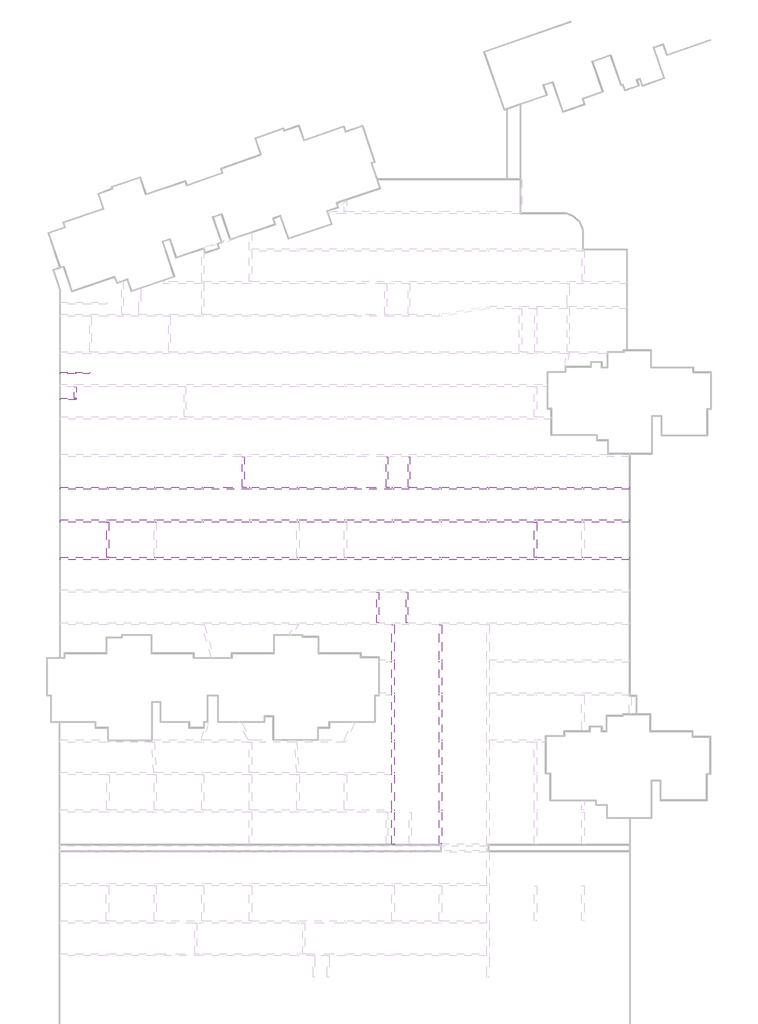
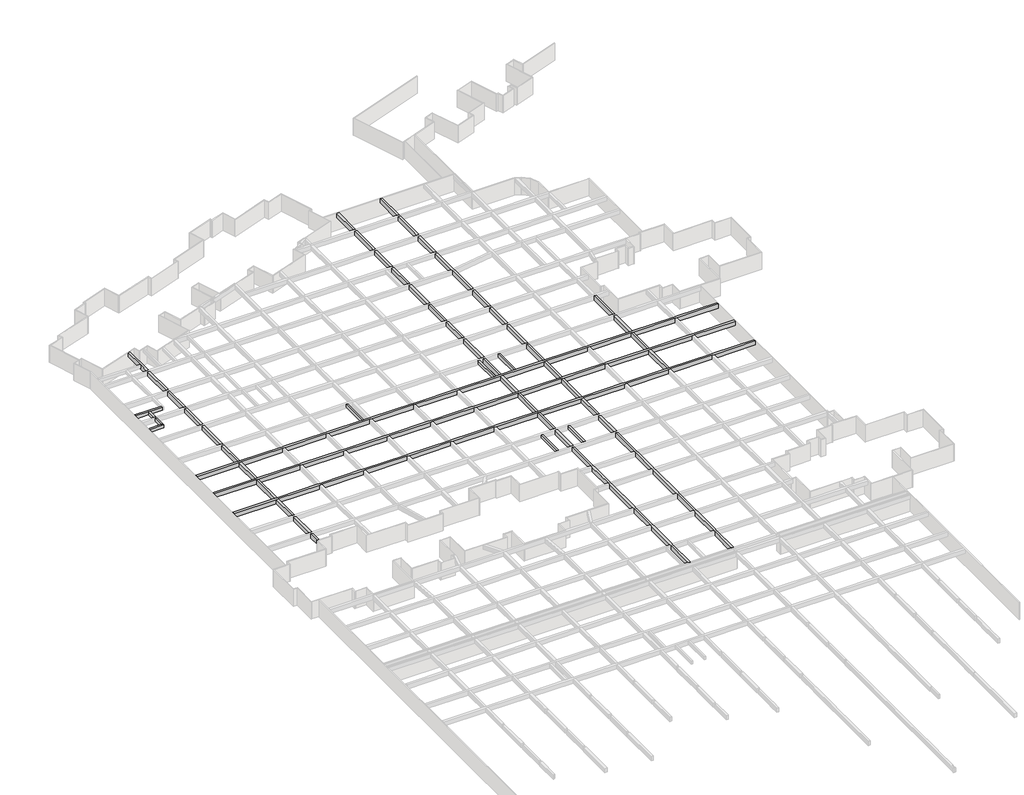
# One storey, part 12 of 14: 15 beams.
"""IFC4 building model written with IfcOpenShell, lengths in millimetres."""

from ifc_helpers import new_model, si_unit, frame, origin, place, context, project, spatial, polyline, outline, extrude, faceted_brep, element, save

model = new_model("IFC4")

# Units and contexts
model_context = context("Model", 3, world=origin())
ifc_project = project(units=[si_unit("LENGTHUNIT", "METRE", prefix="MILLI")], contexts=[model_context])

# Site, building, storey
site = spatial("IfcSite", under=ifc_project)
building = spatial("IfcBuilding", under=site)
storey = spatial("IfcBuildingStorey", under=building, Name="户型图", Elevation=0.0)

# Beams
placement = place(None, origin())
element("IfcBeam", 1, ObjectType="混凝土 - 矩形梁 : KL_beam", at=placement, inside=storey, context=model_context, shape_type="Brep", body=[
    faceted_brep([(-594019.2557706, -67959.4327531, 3300.0), (-594019.2557706, -68359.4327531, 3300.0), (-586267.6529954, -68359.4327531, 3300.0), (-585867.6529954, -68359.4327531, 3300.0), (-578267.6529954, -68359.4327531, 3300.0), (-577867.6529954, -68359.4327531, 3300.0), (-570267.6529954, -68359.4327531, 3300.0), (-569867.6529954, -68359.4327531, 3300.0), (-562267.6529954, -68359.4327531, 3300.0), (-561867.6529954, -68359.4327531, 3300.0), (-554267.6529954, -68359.4327531, 3300.0), (-553867.6529954, -68359.4327531, 3300.0), (-546267.6529954, -68359.4327531, 3300.0), (-545867.6529954, -68359.4327531, 3300.0), (-538267.6529954, -68359.4327531, 3300.0), (-537867.6529954, -68359.4327531, 3300.0), (-530267.6529954, -68359.4327531, 3300.0), (-529867.6529954, -68359.4327531, 3300.0), (-522267.6529954, -68359.4327531, 3300.0), (-521867.6529954, -68359.4327531, 3300.0), (-514267.6529954, -68359.4327531, 3300.0), (-513867.6529954, -68359.4327531, 3300.0), (-506267.6529954, -68359.4327531, 3300.0), (-505867.6529954, -68359.4327531, 3300.0), (-498277.6529954, -68359.4327531, 3300.0), (-498277.6529954, -67959.4327531, 3300.0), (-505867.6529954, -67959.4327531, 3300.0), (-506267.6529954, -67959.4327531, 3300.0), (-513867.6529954, -67959.4327531, 3300.0), (-514267.6529954, -67959.4327531, 3300.0), (-521867.6529954, -67959.4327531, 3300.0), (-522267.6529954, -67959.4327531, 3300.0), (-529867.6529954, -67959.4327531, 3300.0), (-530267.6529954, -67959.4327531, 3300.0), (-535217.6529954, -67959.4327531, 3300.0), (-535517.6529954, -67959.4327531, 3300.0), (-537867.6529954, -67959.4327531, 3300.0), (-538267.6529954, -67959.4327531, 3300.0), (-538917.6529954, -67959.4327531, 3300.0), (-539217.6529954, -67959.4327531, 3300.0), (-545867.6529954, -67959.4327531, 3300.0), (-546267.6529954, -67959.4327531, 3300.0), (-553867.6529954, -67959.4327531, 3300.0), (-554267.6529954, -67959.4327531, 3300.0), (-561867.6529954, -67959.4327531, 3300.0), (-562267.6529954, -67959.4327531, 3300.0), (-563117.6529954, -67959.4327531, 3300.0), (-563417.6529954, -67959.4327531, 3300.0), (-569867.6529954, -67959.4327531, 3300.0), (-570267.6529954, -67959.4327531, 3300.0), (-577867.6529954, -67959.4327531, 3300.0), (-578267.6529954, -67959.4327531, 3300.0), (-585867.6529954, -67959.4327531, 3300.0), (-586267.6529954, -67959.4327531, 3300.0), (-594019.2557706, -67959.4327531, 2500.0), (-498277.6529954, -67959.4327531, 2500.0), (-505867.6529954, -67959.4327531, 2500.0), (-506267.6529954, -67959.4327531, 2500.0), (-513867.6529954, -67959.4327531, 2500.0), (-514267.6529954, -67959.4327531, 2500.0), (-521867.6529954, -67959.4327531, 2500.0), (-522267.6529954, -67959.4327531, 2500.0), (-529867.6529954, -67959.4327531, 2500.0), (-530267.6529954, -67959.4327531, 2500.0), (-537867.6529954, -67959.4327531, 2500.0), (-538267.6529954, -67959.4327531, 2500.0), (-545867.6529954, -67959.4327531, 2500.0), (-546267.6529954, -67959.4327531, 2500.0), (-553867.6529954, -67959.4327531, 2500.0), (-554267.6529954, -67959.4327531, 2500.0), (-561867.6529954, -67959.4327531, 2500.0), (-562267.6529954, -67959.4327531, 2500.0), (-569867.6529954, -67959.4327531, 2500.0), (-570267.6529954, -67959.4327531, 2500.0), (-577867.6529954, -67959.4327531, 2500.0), (-578267.6529954, -67959.4327531, 2500.0), (-585867.6529954, -67959.4327531, 2500.0), (-586267.6529954, -67959.4327531, 2500.0), (-594019.2557706, -68359.4327531, 2500.0), (-498277.6529954, -68359.4327531, 2500.0), (-505867.6529954, -68359.4327531, 2500.0), (-506267.6529954, -68359.4327531, 2500.0), (-513867.6529954, -68359.4327531, 2500.0), (-514267.6529954, -68359.4327531, 2500.0), (-521867.6529954, -68359.4327531, 2500.0), (-522267.6529954, -68359.4327531, 2500.0), (-529867.6529954, -68359.4327531, 2500.0), (-530267.6529954, -68359.4327531, 2500.0), (-537867.6529954, -68359.4327531, 2500.0), (-538267.6529954, -68359.4327531, 2500.0), (-545867.6529954, -68359.4327531, 2500.0), (-546267.6529954, -68359.4327531, 2500.0), (-553867.6529954, -68359.4327531, 2500.0), (-554267.6529954, -68359.4327531, 2500.0), (-561867.6529954, -68359.4327531, 2500.0), (-562267.6529954, -68359.4327531, 2500.0), (-569867.6529954, -68359.4327531, 2500.0), (-570267.6529954, -68359.4327531, 2500.0), (-577867.6529954, -68359.4327531, 2500.0), (-578267.6529954, -68359.4327531, 2500.0), (-585867.6529954, -68359.4327531, 2500.0), (-586267.6529954, -68359.4327531, 2500.0)], [[[0, 1, 2, 3, 4, 5, 6, 7, 8, 9, 10, 11, 12, 13, 14, 15, 16, 17, 18, 19, 20, 21, 22, 23, 24, 25, 26, 27, 28, 29, 30, 31, 32, 33, 34, 35, 36, 37, 38, 39, 40, 41, 42, 43, 44, 45, 46, 47, 48, 49, 50, 51, 52, 53]], [[54, 0, 53, 52, 51, 50, 49, 48, 47, 46, 45, 44, 43, 42, 41, 40, 39, 38, 37, 36, 35, 34, 33, 32, 31, 30, 29, 28, 27, 26, 25, 55, 56, 57, 58, 59, 60, 61, 62, 63, 64, 65, 66, 67, 68, 69, 70, 71, 72, 73, 74, 75, 76, 77]], [[78, 54, 77, 76, 75, 74, 73, 72, 71, 70, 69, 68, 67, 66, 65, 64, 63, 62, 61, 60, 59, 58, 57, 56, 55, 79, 80, 81, 82, 83, 84, 85, 86, 87, 88, 89, 90, 91, 92, 93, 94, 95, 96, 97, 98, 99, 100, 101]], [[1, 78, 101, 100, 99, 98, 97, 96, 95, 94, 93, 92, 91, 90, 89, 88, 87, 86, 85, 84, 83, 82, 81, 80, 79, 24, 23, 22, 21, 20, 19, 18, 17, 16, 15, 14, 13, 12, 11, 10, 9, 8, 7, 6, 5, 4, 3, 2]], [[1, 0, 54, 78]], [[25, 24, 79, 55]]]),
])
element("IfcBeam", 2, ObjectType="混凝土 - 矩形梁 : KL_beam", at=placement, inside=storey, context=model_context, shape_type="Brep", body=[
    faceted_brep([(-594019.2557706, -73459.4327531, 3300.0), (-594019.2557706, -73859.4327531, 3300.0), (-586267.6529954, -73859.4327531, 3300.0), (-585867.6529954, -73859.4327531, 3300.0), (-578267.6529954, -73859.4327531, 3300.0), (-577867.6529954, -73859.4327531, 3300.0), (-570267.6529954, -73859.4327531, 3300.0), (-569867.6529954, -73859.4327531, 3300.0), (-562267.6529954, -73859.4327531, 3300.0), (-561867.6529954, -73859.4327531, 3300.0), (-554267.6529954, -73859.4327531, 3300.0), (-553867.6529954, -73859.4327531, 3300.0), (-546267.6529954, -73859.4327531, 3300.0), (-545867.6529954, -73859.4327531, 3300.0), (-538267.6529954, -73859.4327531, 3300.0), (-537867.6529954, -73859.4327531, 3300.0), (-530267.6529954, -73859.4327531, 3300.0), (-529867.6529954, -73859.4327531, 3300.0), (-522267.6529954, -73859.4327531, 3300.0), (-521867.6529954, -73859.4327531, 3300.0), (-514267.6529954, -73859.4327531, 3300.0), (-513867.6529954, -73859.4327531, 3300.0), (-506267.6529954, -73859.4327531, 3300.0), (-505867.6529954, -73859.4327531, 3300.0), (-498277.6529954, -73859.4327531, 3300.0), (-498277.6529954, -73459.4327531, 3300.0), (-505867.6529954, -73459.4327531, 3300.0), (-506267.6529954, -73459.4327531, 3300.0), (-513867.6529954, -73459.4327531, 3300.0), (-514267.6529954, -73459.4327531, 3300.0), (-521867.6529954, -73459.4327531, 3300.0), (-522267.6529954, -73459.4327531, 3300.0), (-529867.6529954, -73459.4327531, 3300.0), (-530267.6529954, -73459.4327531, 3300.0), (-537867.6529954, -73459.4327531, 3300.0), (-538267.6529954, -73459.4327531, 3300.0), (-545867.6529954, -73459.4327531, 3300.0), (-546267.6529954, -73459.4327531, 3300.0), (-553867.6529954, -73459.4327531, 3300.0), (-554267.6529954, -73459.4327531, 3300.0), (-561867.6529954, -73459.4327531, 3300.0), (-562267.6529954, -73459.4327531, 3300.0), (-569867.6529954, -73459.4327531, 3300.0), (-570267.6529954, -73459.4327531, 3300.0), (-577867.6529954, -73459.4327531, 3300.0), (-578267.6529954, -73459.4327531, 3300.0), (-585867.6529954, -73459.4327531, 3300.0), (-586267.6529954, -73459.4327531, 3300.0), (-594019.2557706, -73859.4327531, 2500.0), (-586267.6529954, -73859.4327531, 2500.0), (-585867.6529954, -73859.4327531, 2500.0), (-578267.6529954, -73859.4327531, 2500.0), (-577867.6529954, -73859.4327531, 2500.0), (-570267.6529954, -73859.4327531, 2500.0), (-569867.6529954, -73859.4327531, 2500.0), (-562267.6529954, -73859.4327531, 2500.0), (-561867.6529954, -73859.4327531, 2500.0), (-554267.6529954, -73859.4327531, 2500.0), (-553867.6529954, -73859.4327531, 2500.0), (-546267.6529954, -73859.4327531, 2500.0), (-545867.6529954, -73859.4327531, 2500.0), (-538267.6529954, -73859.4327531, 2500.0), (-537867.6529954, -73859.4327531, 2500.0), (-530267.6529954, -73859.4327531, 2500.0), (-529867.6529954, -73859.4327531, 2500.0), (-522267.6529954, -73859.4327531, 2500.0), (-521867.6529954, -73859.4327531, 2500.0), (-514267.6529954, -73859.4327531, 2500.0), (-513867.6529954, -73859.4327531, 2500.0), (-506267.6529954, -73859.4327531, 2500.0), (-505867.6529954, -73859.4327531, 2500.0), (-498277.6529954, -73859.4327531, 2500.0), (-594019.2557706, -73459.4327531, 2500.0), (-586267.6529954, -73459.4327531, 2500.0), (-585867.6529954, -73459.4327531, 2500.0), (-578267.6529954, -73459.4327531, 2500.0), (-577867.6529954, -73459.4327531, 2500.0), (-570267.6529954, -73459.4327531, 2500.0), (-569867.6529954, -73459.4327531, 2500.0), (-562267.6529954, -73459.4327531, 2500.0), (-561867.6529954, -73459.4327531, 2500.0), (-554267.6529954, -73459.4327531, 2500.0), (-553867.6529954, -73459.4327531, 2500.0), (-546267.6529954, -73459.4327531, 2500.0), (-545867.6529954, -73459.4327531, 2500.0), (-538267.6529954, -73459.4327531, 2500.0), (-537867.6529954, -73459.4327531, 2500.0), (-530267.6529954, -73459.4327531, 2500.0), (-529867.6529954, -73459.4327531, 2500.0), (-522267.6529954, -73459.4327531, 2500.0), (-521867.6529954, -73459.4327531, 2500.0), (-514267.6529954, -73459.4327531, 2500.0), (-513867.6529954, -73459.4327531, 2500.0), (-506267.6529954, -73459.4327531, 2500.0), (-505867.6529954, -73459.4327531, 2500.0), (-498277.6529954, -73459.4327531, 2500.0)], [[[0, 1, 2, 3, 4, 5, 6, 7, 8, 9, 10, 11, 12, 13, 14, 15, 16, 17, 18, 19, 20, 21, 22, 23, 24, 25, 26, 27, 28, 29, 30, 31, 32, 33, 34, 35, 36, 37, 38, 39, 40, 41, 42, 43, 44, 45, 46, 47]], [[1, 48, 49, 50, 51, 52, 53, 54, 55, 56, 57, 58, 59, 60, 61, 62, 63, 64, 65, 66, 67, 68, 69, 70, 71, 24, 23, 22, 21, 20, 19, 18, 17, 16, 15, 14, 13, 12, 11, 10, 9, 8, 7, 6, 5, 4, 3, 2]], [[48, 72, 73, 74, 75, 76, 77, 78, 79, 80, 81, 82, 83, 84, 85, 86, 87, 88, 89, 90, 91, 92, 93, 94, 95, 71, 70, 69, 68, 67, 66, 65, 64, 63, 62, 61, 60, 59, 58, 57, 56, 55, 54, 53, 52, 51, 50, 49]], [[72, 0, 47, 46, 45, 44, 43, 42, 41, 40, 39, 38, 37, 36, 35, 34, 33, 32, 31, 30, 29, 28, 27, 26, 25, 95, 94, 93, 92, 91, 90, 89, 88, 87, 86, 85, 84, 83, 82, 81, 80, 79, 78, 77, 76, 75, 74, 73]], [[1, 0, 72, 48]], [[25, 24, 71, 95]]]),
])
element("IfcBeam", 3, ObjectType="混凝土 - 矩形梁 : KL_beam", at=placement, inside=storey, context=model_context, shape_type="Brep", body=[
    faceted_brep([(-594019.2557706, -79759.4327531, 3300.0), (-594019.2557706, -80159.4327531, 3300.0), (-586267.6529954, -80159.4327531, 3300.0), (-585867.6529954, -80159.4327531, 3300.0), (-578267.6529954, -80159.4327531, 3300.0), (-577867.6529954, -80159.4327531, 3300.0), (-570267.6529954, -80159.4327531, 3300.0), (-569867.6529954, -80159.4327531, 3300.0), (-562267.6529954, -80159.4327531, 3300.0), (-561867.6529954, -80159.4327531, 3300.0), (-554267.6529954, -80159.4327531, 3300.0), (-553867.6529954, -80159.4327531, 3300.0), (-546267.6529954, -80159.4327531, 3300.0), (-545867.6529954, -80159.4327531, 3300.0), (-538267.6529954, -80159.4327531, 3300.0), (-537867.6529954, -80159.4327531, 3300.0), (-530267.6529954, -80159.4327531, 3300.0), (-529867.6529954, -80159.4327531, 3300.0), (-522267.6529954, -80159.4327531, 3300.0), (-521867.6529954, -80159.4327531, 3300.0), (-514267.6529954, -80159.4327531, 3300.0), (-513867.6529954, -80159.4327531, 3300.0), (-506267.6529954, -80159.4327531, 3300.0), (-505867.6529954, -80159.4327531, 3300.0), (-498277.6529954, -80159.4327531, 3300.0), (-498277.6529954, -79759.4327531, 3300.0), (-505867.6529954, -79759.4327531, 3300.0), (-506267.6529954, -79759.4327531, 3300.0), (-513867.6529954, -79759.4327531, 3300.0), (-514267.6529954, -79759.4327531, 3300.0), (-521867.6529954, -79759.4327531, 3300.0), (-522267.6529954, -79759.4327531, 3300.0), (-529867.6529954, -79759.4327531, 3300.0), (-530267.6529954, -79759.4327531, 3300.0), (-537867.6529954, -79759.4327531, 3300.0), (-538267.6529954, -79759.4327531, 3300.0), (-545867.6529954, -79759.4327531, 3300.0), (-546267.6529954, -79759.4327531, 3300.0), (-553867.6529954, -79759.4327531, 3300.0), (-554267.6529954, -79759.4327531, 3300.0), (-561867.6529954, -79759.4327531, 3300.0), (-562267.6529954, -79759.4327531, 3300.0), (-569867.6529954, -79759.4327531, 3300.0), (-570267.6529954, -79759.4327531, 3300.0), (-577867.6529954, -79759.4327531, 3300.0), (-578267.6529954, -79759.4327531, 3300.0), (-585867.6529954, -79759.4327531, 3300.0), (-586267.6529954, -79759.4327531, 3300.0), (-594019.2557706, -79759.4327531, 2500.0), (-498277.6529954, -79759.4327531, 2500.0), (-505867.6529954, -79759.4327531, 2500.0), (-506267.6529954, -79759.4327531, 2500.0), (-513867.6529954, -79759.4327531, 2500.0), (-514267.6529954, -79759.4327531, 2500.0), (-521867.6529954, -79759.4327531, 2500.0), (-522267.6529954, -79759.4327531, 2500.0), (-529867.6529954, -79759.4327531, 2500.0), (-530267.6529954, -79759.4327531, 2500.0), (-537867.6529954, -79759.4327531, 2500.0), (-538267.6529954, -79759.4327531, 2500.0), (-545867.6529954, -79759.4327531, 2500.0), (-546267.6529954, -79759.4327531, 2500.0), (-553867.6529954, -79759.4327531, 2500.0), (-554267.6529954, -79759.4327531, 2500.0), (-561867.6529954, -79759.4327531, 2500.0), (-562267.6529954, -79759.4327531, 2500.0), (-569867.6529954, -79759.4327531, 2500.0), (-570267.6529954, -79759.4327531, 2500.0), (-577867.6529954, -79759.4327531, 2500.0), (-578267.6529954, -79759.4327531, 2500.0), (-585867.6529954, -79759.4327531, 2500.0), (-586267.6529954, -79759.4327531, 2500.0), (-594019.2557706, -80159.4327531, 2500.0), (-498277.6529954, -80159.4327531, 2500.0), (-505867.6529954, -80159.4327531, 2500.0), (-506267.6529954, -80159.4327531, 2500.0), (-513867.6529954, -80159.4327531, 2500.0), (-514267.6529954, -80159.4327531, 2500.0), (-521867.6529954, -80159.4327531, 2500.0), (-522267.6529954, -80159.4327531, 2500.0), (-529867.6529954, -80159.4327531, 2500.0), (-530267.6529954, -80159.4327531, 2500.0), (-537867.6529954, -80159.4327531, 2500.0), (-538267.6529954, -80159.4327531, 2500.0), (-545867.6529954, -80159.4327531, 2500.0), (-546267.6529954, -80159.4327531, 2500.0), (-553867.6529954, -80159.4327531, 2500.0), (-554267.6529954, -80159.4327531, 2500.0), (-561867.6529954, -80159.4327531, 2500.0), (-562267.6529954, -80159.4327531, 2500.0), (-569867.6529954, -80159.4327531, 2500.0), (-570267.6529954, -80159.4327531, 2500.0), (-577867.6529954, -80159.4327531, 2500.0), (-578267.6529954, -80159.4327531, 2500.0), (-585867.6529954, -80159.4327531, 2500.0), (-586267.6529954, -80159.4327531, 2500.0)], [[[0, 1, 2, 3, 4, 5, 6, 7, 8, 9, 10, 11, 12, 13, 14, 15, 16, 17, 18, 19, 20, 21, 22, 23, 24, 25, 26, 27, 28, 29, 30, 31, 32, 33, 34, 35, 36, 37, 38, 39, 40, 41, 42, 43, 44, 45, 46, 47]], [[48, 0, 47, 46, 45, 44, 43, 42, 41, 40, 39, 38, 37, 36, 35, 34, 33, 32, 31, 30, 29, 28, 27, 26, 25, 49, 50, 51, 52, 53, 54, 55, 56, 57, 58, 59, 60, 61, 62, 63, 64, 65, 66, 67, 68, 69, 70, 71]], [[72, 48, 71, 70, 69, 68, 67, 66, 65, 64, 63, 62, 61, 60, 59, 58, 57, 56, 55, 54, 53, 52, 51, 50, 49, 73, 74, 75, 76, 77, 78, 79, 80, 81, 82, 83, 84, 85, 86, 87, 88, 89, 90, 91, 92, 93, 94, 95]], [[1, 72, 95, 94, 93, 92, 91, 90, 89, 88, 87, 86, 85, 84, 83, 82, 81, 80, 79, 78, 77, 76, 75, 74, 73, 24, 23, 22, 21, 20, 19, 18, 17, 16, 15, 14, 13, 12, 11, 10, 9, 8, 7, 6, 5, 4, 3, 2]], [[1, 0, 48, 72]], [[25, 24, 73, 49]]]),
])
element("IfcBeam", 4, ObjectType="混凝土 - 矩形梁 : KL_beam", at=placement, inside=storey, context=model_context, shape_type="Brep", body=[
    faceted_brep([(-585867.6529954, -33000.9936522, 3300.0), (-586267.6529954, -33135.1346091, 3300.0), (-586267.6529954, -36909.4327532, 3300.0), (-586267.6529954, -37209.4327532, 3300.0), (-586267.6529954, -38859.4327531, 3300.0), (-585867.6529954, -38859.4327531, 3300.0), (-585867.6529954, -33000.9936522, 2500.0), (-585867.6529954, -38859.4327531, 2500.0), (-586267.6529954, -33135.1346091, 2500.0), (-586267.6529954, -38859.4327531, 2500.0)], [[[0, 1, 2, 3, 4, 5]], [[6, 0, 5, 7]], [[8, 6, 7, 9]], [[1, 8, 9, 4, 3, 2]], [[1, 0, 6, 8]], [[5, 4, 9, 7]]]),
    faceted_brep([(-585867.6529954, -93205.835545, 3300.0), (-586267.6529954, -93205.835545, 3300.0), (-586267.6529954, -93205.835545, 2500.0), (-585867.6529954, -93205.835545, 2500.0), (-586267.6529954, -91159.4327531, 3300.0), (-585867.6529954, -91159.4327531, 3300.0), (-585867.6529954, -91159.4327531, 2500.0), (-586267.6529954, -91159.4327531, 2500.0)], [[[0, 1, 2, 3]], [[4, 5, 6, 7]], [[1, 0, 5, 4]], [[0, 3, 6, 5]], [[3, 2, 7, 6]], [[2, 1, 4, 7]]]),
    faceted_brep([(-586267.6529954, -39259.4327531, 3300.0), (-585867.6529954, -39259.4327531, 3300.0), (-585867.6529954, -39259.4327531, 2500.0), (-586267.6529954, -39259.4327531, 2500.0), (-586267.6529954, -45159.4327531, 3300.0), (-585867.6529954, -45159.4327531, 3300.0), (-585867.6529954, -45159.4327531, 2500.0), (-586267.6529954, -45159.4327531, 2500.0)], [[[0, 1, 2, 3]], [[1, 0, 4, 5]], [[2, 1, 5, 6]], [[3, 2, 6, 7]], [[0, 3, 7, 4]], [[5, 4, 7, 6]]]),
    faceted_brep([(-586267.6529954, -45559.4327531, 3300.0), (-585867.6529954, -45559.4327531, 3300.0), (-585867.6529954, -45559.4327531, 2500.0), (-586267.6529954, -45559.4327531, 2500.0), (-586267.6529954, -50659.4327531, 3300.0), (-585867.6529954, -50659.4327531, 3300.0), (-585867.6529954, -50659.4327531, 2500.0), (-586267.6529954, -50659.4327531, 2500.0)], [[[0, 1, 2, 3]], [[1, 0, 4, 5]], [[2, 1, 5, 6]], [[3, 2, 6, 7]], [[0, 3, 7, 4]], [[5, 4, 7, 6]]]),
    faceted_brep([(-586267.6529954, -56559.4327531, 3300.0), (-585867.6529954, -56559.4327531, 3300.0), (-585867.6529954, -56559.4327531, 2500.0), (-586267.6529954, -56559.4327531, 2500.0), (-586267.6529954, -62459.4327531, 3300.0), (-585867.6529954, -62459.4327531, 3300.0), (-585867.6529954, -62459.4327531, 2500.0), (-586267.6529954, -62459.4327531, 2500.0)], [[[0, 1, 2, 3]], [[1, 0, 4, 5]], [[2, 1, 5, 6]], [[3, 2, 6, 7]], [[0, 3, 7, 4]], [[5, 4, 7, 6]]]),
    faceted_brep([(-585867.6529954, -56159.4327531, 3300.0), (-586267.6529954, -56159.4327531, 3300.0), (-586267.6529954, -56159.4327531, 2500.0), (-585867.6529954, -56159.4327531, 2500.0), (-586267.6529954, -51059.4327531, 3300.0), (-585867.6529954, -51059.4327531, 3300.0), (-585867.6529954, -51059.4327531, 2500.0), (-586267.6529954, -51059.4327531, 2500.0)], [[[0, 1, 2, 3]], [[4, 5, 6, 7]], [[1, 0, 5, 4]], [[0, 3, 6, 5]], [[3, 2, 7, 6]], [[2, 1, 4, 7]]]),
    faceted_brep([(-586267.6529954, -62859.4327531, 3300.0), (-585867.6529954, -62859.4327531, 3300.0), (-585867.6529954, -62859.4327531, 2500.0), (-586267.6529954, -62859.4327531, 2500.0), (-586267.6529954, -67959.4327531, 3300.0), (-585867.6529954, -67959.4327531, 3300.0), (-585867.6529954, -67959.4327531, 2500.0), (-586267.6529954, -67959.4327531, 2500.0)], [[[0, 1, 2, 3]], [[1, 0, 4, 5]], [[2, 1, 5, 6]], [[3, 2, 6, 7]], [[0, 3, 7, 4]], [[5, 4, 7, 6]]]),
    faceted_brep([(-586267.6529954, -68359.4327531, 3300.0), (-585867.6529954, -68359.4327531, 3300.0), (-585867.6529954, -68359.4327531, 2500.0), (-586267.6529954, -68359.4327531, 2500.0), (-586267.6529954, -73459.4327531, 3300.0), (-585867.6529954, -73459.4327531, 3300.0), (-585867.6529954, -73459.4327531, 2500.0), (-586267.6529954, -73459.4327531, 2500.0)], [[[0, 1, 2, 3]], [[1, 0, 4, 5]], [[2, 1, 5, 6]], [[3, 2, 6, 7]], [[0, 3, 7, 4]], [[5, 4, 7, 6]]]),
    faceted_brep([(-586267.6529954, -73859.4327531, 3300.0), (-585867.6529954, -73859.4327531, 3300.0), (-585867.6529954, -73859.4327531, 2500.0), (-586267.6529954, -73859.4327531, 2500.0), (-586267.6529954, -79759.4327531, 3300.0), (-585867.6529954, -79759.4327531, 3300.0), (-585867.6529954, -79759.4327531, 2500.0), (-586267.6529954, -79759.4327531, 2500.0)], [[[0, 1, 2, 3]], [[1, 0, 4, 5]], [[2, 1, 5, 6]], [[3, 2, 6, 7]], [[0, 3, 7, 4]], [[5, 4, 7, 6]]]),
    faceted_brep([(-586267.6529954, -80159.4327531, 3300.0), (-585867.6529954, -80159.4327531, 3300.0), (-585867.6529954, -80159.4327531, 2500.0), (-586267.6529954, -80159.4327531, 2500.0), (-586267.6529954, -85259.4327531, 3300.0), (-585867.6529954, -85259.4327531, 3300.0), (-585867.6529954, -85259.4327531, 2500.0), (-586267.6529954, -85259.4327531, 2500.0)], [[[0, 1, 2, 3]], [[1, 0, 4, 5]], [[2, 1, 5, 6]], [[3, 2, 6, 7]], [[0, 3, 7, 4]], [[5, 4, 7, 6]]]),
    faceted_brep([(-586267.6529954, -85659.4327531, 3300.0), (-585867.6529954, -85659.4327531, 3300.0), (-585867.6529954, -85659.4327531, 2500.0), (-586267.6529954, -85659.4327531, 2500.0), (-586267.6529954, -90759.4327531, 3300.0), (-585867.6529954, -90759.4327531, 3300.0), (-585867.6529954, -90759.4327531, 2500.0), (-586267.6529954, -90759.4327531, 2500.0)], [[[0, 1, 2, 3]], [[1, 0, 4, 5]], [[2, 1, 5, 6]], [[3, 2, 6, 7]], [[0, 3, 7, 4]], [[5, 4, 7, 6]]]),
])
element("IfcBeam", 5, ObjectType="混凝土 - 矩形梁 : KL_beam", at=placement, inside=storey, context=model_context, shape_type="Brep", body=[
    faceted_brep([(-537867.6529954, -16219.4327531, 3300.0), (-538267.6529954, -16219.4327531, 3300.0), (-538267.6529954, -21559.4327531, 3300.0), (-537867.6529954, -21559.4327531, 3300.0), (-538267.6529954, -16219.4327531, 2500.0), (-538267.6529954, -21559.4327531, 2500.0), (-537867.6529954, -16219.4327531, 2500.0), (-537867.6529954, -21559.4327531, 2500.0)], [[[0, 1, 2, 3]], [[1, 4, 5, 2]], [[4, 6, 7, 5]], [[6, 0, 3, 7]], [[1, 0, 6, 4]], [[3, 2, 5, 7]]]),
    faceted_brep([(-537867.6529954, -128099.4327532, 3300.0), (-538267.6529954, -128099.4327532, 3300.0), (-538267.6529954, -128099.4327532, 2500.0), (-537867.6529954, -128099.4327532, 2500.0), (-537867.6529954, -127959.4327532, 3300.0), (-537867.6529954, -122659.4327531, 3300.0), (-537867.6529954, -122259.4327531, 3300.0), (-537867.6529954, -116357.5126628, 3300.0), (-537867.6529954, -115957.5126628, 3300.0), (-537867.6529954, -110859.4327531, 3300.0), (-537867.6529954, -110459.4327531, 3300.0), (-537867.6529954, -102959.4327531, 3300.0), (-537867.6529954, -102559.4327531, 3300.0), (-537867.6529954, -97459.4327531, 3300.0), (-537867.6529954, -97059.4327531, 3300.0), (-537867.6529954, -91159.4327531, 3300.0), (-538267.6529954, -91159.4327531, 3300.0), (-538267.6529954, -97059.4327531, 3300.0), (-538267.6529954, -97459.4327531, 3300.0), (-538267.6529954, -102559.4327531, 3300.0), (-538267.6529954, -102959.4327531, 3300.0), (-538267.6529954, -110459.4327531, 3300.0), (-538267.6529954, -110859.4327531, 3300.0), (-538267.6529954, -115957.5126628, 3300.0), (-538267.6529954, -116357.5126628, 3300.0), (-538267.6529954, -122259.4327531, 3300.0), (-538267.6529954, -122659.4327531, 3300.0), (-538267.6529954, -127959.4327532, 3300.0), (-538267.6529954, -91159.4327531, 2500.0), (-538267.6529954, -97059.4327531, 2500.0), (-538267.6529954, -97459.4327531, 2500.0), (-538267.6529954, -102559.4327531, 2500.0), (-538267.6529954, -102959.4327531, 2500.0), (-538267.6529954, -110459.4327531, 2500.0), (-538267.6529954, -110859.4327531, 2500.0), (-538267.6529954, -115957.5126628, 2500.0), (-538267.6529954, -116357.5126628, 2500.0), (-538267.6529954, -122259.4327531, 2500.0), (-538267.6529954, -122659.4327531, 2500.0), (-538267.6529954, -127959.4327532, 2500.0), (-537867.6529954, -91159.4327531, 2500.0), (-537867.6529954, -97059.4327531, 2500.0), (-537867.6529954, -97459.4327531, 2500.0), (-537867.6529954, -102559.4327531, 2500.0), (-537867.6529954, -102959.4327531, 2500.0), (-537867.6529954, -110459.4327531, 2500.0), (-537867.6529954, -110859.4327531, 2500.0), (-537867.6529954, -115957.5126628, 2500.0), (-537867.6529954, -116357.5126628, 2500.0), (-537867.6529954, -122259.4327531, 2500.0), (-537867.6529954, -122659.4327531, 2500.0), (-537867.6529954, -127959.4327532, 2500.0)], [[[0, 1, 2, 3]], [[1, 0, 4, 5, 6, 7, 8, 9, 10, 11, 12, 13, 14, 15, 16, 17, 18, 19, 20, 21, 22, 23, 24, 25, 26, 27]], [[2, 1, 27, 26, 25, 24, 23, 22, 21, 20, 19, 18, 17, 16, 28, 29, 30, 31, 32, 33, 34, 35, 36, 37, 38, 39]], [[3, 2, 39, 38, 37, 36, 35, 34, 33, 32, 31, 30, 29, 28, 40, 41, 42, 43, 44, 45, 46, 47, 48, 49, 50, 51]], [[0, 3, 51, 50, 49, 48, 47, 46, 45, 44, 43, 42, 41, 40, 15, 14, 13, 12, 11, 10, 9, 8, 7, 6, 5, 4]], [[16, 15, 40, 28]]]),
    faceted_brep([(-538267.6529954, -33759.4327531, 3300.0), (-537867.6529954, -33759.4327531, 3300.0), (-537867.6529954, -33759.4327531, 2500.0), (-538267.6529954, -33759.4327531, 2500.0), (-537867.6529954, -38859.4327531, 3300.0), (-538267.6529954, -38859.4327531, 3300.0), (-538267.6529954, -38859.4327531, 2500.0), (-537867.6529954, -38859.4327531, 2500.0)], [[[0, 1, 2, 3]], [[4, 5, 6, 7]], [[1, 0, 5, 4]], [[0, 3, 6, 5]], [[3, 2, 7, 6]], [[2, 1, 4, 7]]]),
    faceted_brep([(-537867.6529954, -33359.4327531, 3300.0), (-538267.6529954, -33359.4327531, 3300.0), (-538267.6529954, -33359.4327531, 2500.0), (-537867.6529954, -33359.4327531, 2500.0), (-538267.6529954, -28259.4327531, 3300.0), (-537867.6529954, -28259.4327531, 3300.0), (-537867.6529954, -28259.4327531, 2500.0), (-538267.6529954, -28259.4327531, 2500.0)], [[[0, 1, 2, 3]], [[4, 5, 6, 7]], [[1, 0, 5, 4]], [[2, 1, 4, 7]], [[3, 2, 7, 6]], [[0, 3, 6, 5]]]),
    faceted_brep([(-537867.6529954, -39259.4327531, 3300.0), (-538267.6529954, -39259.4327531, 3300.0), (-538267.6529954, -45159.4327531, 3300.0), (-537867.6529954, -45159.4327531, 3300.0), (-538267.6529954, -39259.4327531, 2500.0), (-538267.6529954, -45159.4327531, 2500.0), (-537867.6529954, -39259.4327531, 2500.0), (-537867.6529954, -45159.4327531, 2500.0)], [[[0, 1, 2, 3]], [[1, 4, 5, 2]], [[4, 6, 7, 5]], [[6, 0, 3, 7]], [[1, 0, 6, 4]], [[3, 2, 5, 7]]]),
    faceted_brep([(-537867.6529954, -27859.4327531, 3300.0), (-538267.6529954, -27859.4327531, 3300.0), (-538267.6529954, -27859.4327531, 2500.0), (-537867.6529954, -27859.4327531, 2500.0), (-538267.6529954, -21959.4327531, 3300.0), (-537867.6529954, -21959.4327531, 3300.0), (-537867.6529954, -21959.4327531, 2500.0), (-538267.6529954, -21959.4327531, 2500.0)], [[[0, 1, 2, 3]], [[4, 5, 6, 7]], [[1, 0, 5, 4]], [[2, 1, 4, 7]], [[3, 2, 7, 6]], [[0, 3, 6, 5]]]),
    faceted_brep([(-538267.6529954, -45559.4327531, 3300.0), (-537867.6529954, -45559.4327531, 3300.0), (-537867.6529954, -45559.4327531, 2500.0), (-538267.6529954, -45559.4327531, 2500.0), (-537867.6529954, -50659.4327531, 3300.0), (-538267.6529954, -50659.4327531, 3300.0), (-538267.6529954, -50659.4327531, 2500.0), (-537867.6529954, -50659.4327531, 2500.0)], [[[0, 1, 2, 3]], [[4, 5, 6, 7]], [[1, 0, 5, 4]], [[0, 3, 6, 5]], [[3, 2, 7, 6]], [[2, 1, 4, 7]]]),
    faceted_brep([(-537867.6529954, -56559.4327531, 3300.0), (-538267.6529954, -56559.4327531, 3300.0), (-538267.6529954, -62459.4327531, 3300.0), (-537867.6529954, -62459.4327531, 3300.0), (-538267.6529954, -56559.4327531, 2500.0), (-538267.6529954, -62459.4327531, 2500.0), (-537867.6529954, -56559.4327531, 2500.0), (-537867.6529954, -62459.4327531, 2500.0)], [[[0, 1, 2, 3]], [[1, 4, 5, 2]], [[4, 6, 7, 5]], [[6, 0, 3, 7]], [[1, 0, 6, 4]], [[3, 2, 5, 7]]]),
    faceted_brep([(-537867.6529954, -56159.4327531, 3300.0), (-538267.6529954, -56159.4327531, 3300.0), (-538267.6529954, -56159.4327531, 2500.0), (-537867.6529954, -56159.4327531, 2500.0), (-537867.6529954, -51059.4327531, 3300.0), (-538267.6529954, -51059.4327531, 3300.0), (-538267.6529954, -51059.4327531, 2500.0), (-537867.6529954, -51059.4327531, 2500.0)], [[[0, 1, 2, 3]], [[1, 0, 4, 5]], [[2, 1, 5, 6]], [[3, 2, 6, 7]], [[0, 3, 7, 4]], [[5, 4, 7, 6]]]),
    faceted_brep([(-538267.6529954, -62859.4327531, 3300.0), (-537867.6529954, -62859.4327531, 3300.0), (-537867.6529954, -62859.4327531, 2500.0), (-538267.6529954, -62859.4327531, 2500.0), (-537867.6529954, -67959.4327531, 3300.0), (-538267.6529954, -67959.4327531, 3300.0), (-538267.6529954, -67959.4327531, 2500.0), (-537867.6529954, -67959.4327531, 2500.0)], [[[0, 1, 2, 3]], [[4, 5, 6, 7]], [[1, 0, 5, 4]], [[0, 3, 6, 5]], [[3, 2, 7, 6]], [[2, 1, 4, 7]]]),
    faceted_brep([(-537867.6529954, -68359.4327531, 3300.0), (-538267.6529954, -68359.4327531, 3300.0), (-538267.6529954, -73459.4327531, 3300.0), (-537867.6529954, -73459.4327531, 3300.0), (-538267.6529954, -68359.4327531, 2500.0), (-538267.6529954, -73459.4327531, 2500.0), (-537867.6529954, -68359.4327531, 2500.0), (-537867.6529954, -73459.4327531, 2500.0)], [[[0, 1, 2, 3]], [[1, 4, 5, 2]], [[4, 6, 7, 5]], [[6, 0, 3, 7]], [[1, 0, 6, 4]], [[3, 2, 5, 7]]]),
    faceted_brep([(-538267.6529954, -73859.4327531, 3300.0), (-537867.6529954, -73859.4327531, 3300.0), (-537867.6529954, -73859.4327531, 2500.0), (-538267.6529954, -73859.4327531, 2500.0), (-537867.6529954, -79759.4327531, 3300.0), (-538267.6529954, -79759.4327531, 3300.0), (-538267.6529954, -79759.4327531, 2500.0), (-537867.6529954, -79759.4327531, 2500.0)], [[[0, 1, 2, 3]], [[4, 5, 6, 7]], [[1, 0, 5, 4]], [[0, 3, 6, 5]], [[3, 2, 7, 6]], [[2, 1, 4, 7]]]),
    faceted_brep([(-537867.6529954, -80159.4327531, 3300.0), (-538267.6529954, -80159.4327531, 3300.0), (-538267.6529954, -85259.4327531, 3300.0), (-537867.6529954, -85259.4327531, 3300.0), (-538267.6529954, -80159.4327531, 2500.0), (-538267.6529954, -85259.4327531, 2500.0), (-537867.6529954, -80159.4327531, 2500.0), (-537867.6529954, -85259.4327531, 2500.0)], [[[0, 1, 2, 3]], [[1, 4, 5, 2]], [[4, 6, 7, 5]], [[6, 0, 3, 7]], [[1, 0, 6, 4]], [[3, 2, 5, 7]]]),
    faceted_brep([(-538267.6529954, -85659.4327531, 3300.0), (-537867.6529954, -85659.4327531, 3300.0), (-537867.6529954, -85659.4327531, 2500.0), (-538267.6529954, -85659.4327531, 2500.0), (-537867.6529954, -90759.4327531, 3300.0), (-538267.6529954, -90759.4327531, 3300.0), (-538267.6529954, -90759.4327531, 2500.0), (-537867.6529954, -90759.4327531, 2500.0)], [[[0, 1, 2, 3]], [[4, 5, 6, 7]], [[1, 0, 5, 4]], [[0, 3, 6, 5]], [[3, 2, 7, 6]], [[2, 1, 4, 7]]]),
])
element("IfcBeam", 6, ObjectType="混凝土 - 矩形梁 : KL_beam", at=placement, inside=storey, context=model_context, shape_type="Brep", body=[
    faceted_brep([(-529867.6529954, -91159.4327531, 3300.0), (-530267.6529954, -91159.4327531, 3300.0), (-530267.6529954, -97059.4327531, 3300.0), (-530267.6529954, -97459.4327531, 3300.0), (-530267.6529954, -102559.4327531, 3300.0), (-530267.6529954, -102959.4327531, 3300.0), (-530267.6529954, -110459.4327531, 3300.0), (-530267.6529954, -110859.4327531, 3300.0), (-530267.6529954, -115957.5126628, 3300.0), (-530267.6529954, -116357.5126628, 3300.0), (-530267.6529954, -122259.4327531, 3300.0), (-530267.6529954, -122659.4327531, 3300.0), (-530267.6529954, -127959.4327532, 3300.0), (-529867.6529954, -127959.4327532, 3300.0), (-529867.6529954, -122659.4327531, 3300.0), (-529867.6529954, -122259.4327531, 3300.0), (-529867.6529954, -116357.5126628, 3300.0), (-529867.6529954, -115957.5126628, 3300.0), (-529867.6529954, -110859.4327531, 3300.0), (-529867.6529954, -110459.4327531, 3300.0), (-529867.6529954, -102959.4327531, 3300.0), (-529867.6529954, -102559.4327531, 3300.0), (-529867.6529954, -97459.4327531, 3300.0), (-529867.6529954, -97059.4327531, 3300.0), (-529867.6529954, -91159.4327531, 2500.0), (-529867.6529954, -127959.4327532, 2500.0), (-529867.6529954, -122659.4327531, 2500.0), (-529867.6529954, -122259.4327531, 2500.0), (-529867.6529954, -116357.5126628, 2500.0), (-529867.6529954, -115957.5126628, 2500.0), (-529867.6529954, -110859.4327531, 2500.0), (-529867.6529954, -110459.4327531, 2500.0), (-529867.6529954, -102959.4327531, 2500.0), (-529867.6529954, -102559.4327531, 2500.0), (-529867.6529954, -97459.4327531, 2500.0), (-529867.6529954, -97059.4327531, 2500.0), (-530267.6529954, -91159.4327531, 2500.0), (-530267.6529954, -127959.4327532, 2500.0), (-530267.6529954, -122659.4327531, 2500.0), (-530267.6529954, -122259.4327531, 2500.0), (-530267.6529954, -116357.5126628, 2500.0), (-530267.6529954, -115957.5126628, 2500.0), (-530267.6529954, -110859.4327531, 2500.0), (-530267.6529954, -110459.4327531, 2500.0), (-530267.6529954, -102959.4327531, 2500.0), (-530267.6529954, -102559.4327531, 2500.0), (-530267.6529954, -97459.4327531, 2500.0), (-530267.6529954, -97059.4327531, 2500.0)], [[[0, 1, 2, 3, 4, 5, 6, 7, 8, 9, 10, 11, 12, 13, 14, 15, 16, 17, 18, 19, 20, 21, 22, 23]], [[24, 0, 23, 22, 21, 20, 19, 18, 17, 16, 15, 14, 13, 25, 26, 27, 28, 29, 30, 31, 32, 33, 34, 35]], [[36, 24, 35, 34, 33, 32, 31, 30, 29, 28, 27, 26, 25, 37, 38, 39, 40, 41, 42, 43, 44, 45, 46, 47]], [[1, 36, 47, 46, 45, 44, 43, 42, 41, 40, 39, 38, 37, 12, 11, 10, 9, 8, 7, 6, 5, 4, 3, 2]], [[1, 0, 24, 36]], [[13, 12, 37, 25]]]),
    faceted_brep([(-530267.6529954, -16219.4327531, 3300.0), (-529867.6529954, -16219.4327531, 3300.0), (-529867.6529954, -16219.4327531, 2500.0), (-530267.6529954, -16219.4327531, 2500.0), (-529867.6529954, -21559.4327531, 3300.0), (-530267.6529954, -21559.4327531, 3300.0), (-530267.6529954, -21559.4327531, 2500.0), (-529867.6529954, -21559.4327531, 2500.0)], [[[0, 1, 2, 3]], [[4, 5, 6, 7]], [[1, 0, 5, 4]], [[2, 1, 4, 7]], [[3, 2, 7, 6]], [[0, 3, 6, 5]]]),
    faceted_brep([(-530267.6529954, -33759.4327531, 3300.0), (-529867.6529954, -33759.4327531, 3300.0), (-529867.6529954, -33759.4327531, 2500.0), (-530267.6529954, -33759.4327531, 2500.0), (-529867.6529954, -45159.4327531, 3300.0), (-530267.6529954, -45159.4327531, 3300.0), (-530267.6529954, -45159.4327531, 2500.0), (-529867.6529954, -45159.4327531, 2500.0), (-530267.6529954, -38859.4327531, 3300.0), (-530267.6529954, -39259.4327531, 3300.0), (-529867.6529954, -39229.5561723, 3300.0), (-529867.6529954, -38824.309334, 3300.0), (-529867.6529954, -39229.5561723, 2500.0), (-529867.6529954, -38824.309334, 2500.0), (-530267.6529954, -39259.4327531, 2500.0), (-530267.6529954, -38859.4327531, 2500.0)], [[[0, 1, 2, 3]], [[4, 5, 6, 7]], [[1, 0, 8, 9, 5, 4, 10, 11]], [[2, 1, 11, 10, 4, 7, 12, 13]], [[3, 2, 13, 12, 7, 6, 14, 15]], [[0, 3, 15, 14, 6, 5, 9, 8]]]),
    faceted_brep([(-529867.6529954, -33359.4327531, 3300.0), (-530267.6529954, -33359.4327531, 3300.0), (-530267.6529954, -33359.4327531, 2500.0), (-529867.6529954, -33359.4327531, 2500.0), (-530267.6529954, -28259.4327531, 3300.0), (-529867.6529954, -28259.4327531, 3300.0), (-529867.6529954, -28259.4327531, 2500.0), (-530267.6529954, -28259.4327531, 2500.0)], [[[0, 1, 2, 3]], [[4, 5, 6, 7]], [[1, 0, 5, 4]], [[0, 3, 6, 5]], [[3, 2, 7, 6]], [[2, 1, 4, 7]]]),
    faceted_brep([(-530267.6529954, -27859.4327531, 3300.0), (-529867.6529954, -27859.4327531, 3300.0), (-529867.6529954, -21959.4327531, 3300.0), (-530267.6529954, -21959.4327531, 3300.0), (-529867.6529954, -27859.4327531, 2500.0), (-529867.6529954, -21959.4327531, 2500.0), (-530267.6529954, -27859.4327531, 2500.0), (-530267.6529954, -21959.4327531, 2500.0)], [[[0, 1, 2, 3]], [[1, 4, 5, 2]], [[4, 6, 7, 5]], [[6, 0, 3, 7]], [[1, 0, 6, 4]], [[3, 2, 5, 7]]]),
    faceted_brep([(-530267.6529954, -45559.4327531, 3300.0), (-529867.6529954, -45559.4327531, 3300.0), (-529867.6529954, -45559.4327531, 2500.0), (-530267.6529954, -45559.4327531, 2500.0), (-529867.6529954, -50659.4327531, 3300.0), (-530267.6529954, -50659.4327531, 3300.0), (-530267.6529954, -50659.4327531, 2500.0), (-529867.6529954, -50659.4327531, 2500.0)], [[[0, 1, 2, 3]], [[4, 5, 6, 7]], [[1, 0, 5, 4]], [[2, 1, 4, 7]], [[3, 2, 7, 6]], [[0, 3, 6, 5]]]),
    faceted_brep([(-530267.6529954, -56559.4327531, 3300.0), (-529867.6529954, -56559.4327531, 3300.0), (-529867.6529954, -56559.4327531, 2500.0), (-530267.6529954, -56559.4327531, 2500.0), (-529867.6529954, -62459.4327531, 3300.0), (-530267.6529954, -62459.4327531, 3300.0), (-530267.6529954, -62459.4327531, 2500.0), (-529867.6529954, -62459.4327531, 2500.0)], [[[0, 1, 2, 3]], [[4, 5, 6, 7]], [[1, 0, 5, 4]], [[2, 1, 4, 7]], [[3, 2, 7, 6]], [[0, 3, 6, 5]]]),
    faceted_brep([(-529867.6529954, -56159.4327531, 3300.0), (-530267.6529954, -56159.4327531, 3300.0), (-530267.6529954, -56159.4327531, 2500.0), (-529867.6529954, -56159.4327531, 2500.0), (-530267.6529954, -51059.4327531, 3300.0), (-529867.6529954, -51059.4327531, 3300.0), (-529867.6529954, -51059.4327531, 2500.0), (-530267.6529954, -51059.4327531, 2500.0)], [[[0, 1, 2, 3]], [[4, 5, 6, 7]], [[1, 0, 5, 4]], [[0, 3, 6, 5]], [[3, 2, 7, 6]], [[2, 1, 4, 7]]]),
    faceted_brep([(-530267.6529954, -62859.4327531, 3300.0), (-529867.6529954, -62859.4327531, 3300.0), (-529867.6529954, -62859.4327531, 2500.0), (-530267.6529954, -62859.4327531, 2500.0), (-529867.6529954, -67959.4327531, 3300.0), (-530267.6529954, -67959.4327531, 3300.0), (-530267.6529954, -67959.4327531, 2500.0), (-529867.6529954, -67959.4327531, 2500.0)], [[[0, 1, 2, 3]], [[4, 5, 6, 7]], [[1, 0, 5, 4]], [[2, 1, 4, 7]], [[3, 2, 7, 6]], [[0, 3, 6, 5]]]),
    faceted_brep([(-530267.6529954, -68359.4327531, 3300.0), (-529867.6529954, -68359.4327531, 3300.0), (-529867.6529954, -68359.4327531, 2500.0), (-530267.6529954, -68359.4327531, 2500.0), (-529867.6529954, -73459.4327531, 3300.0), (-530267.6529954, -73459.4327531, 3300.0), (-530267.6529954, -73459.4327531, 2500.0), (-529867.6529954, -73459.4327531, 2500.0)], [[[0, 1, 2, 3]], [[4, 5, 6, 7]], [[1, 0, 5, 4]], [[2, 1, 4, 7]], [[3, 2, 7, 6]], [[0, 3, 6, 5]]]),
    faceted_brep([(-530267.6529954, -73859.4327531, 3300.0), (-529867.6529954, -73859.4327531, 3300.0), (-529867.6529954, -73859.4327531, 2500.0), (-530267.6529954, -73859.4327531, 2500.0), (-529867.6529954, -79759.4327531, 3300.0), (-530267.6529954, -79759.4327531, 3300.0), (-530267.6529954, -79759.4327531, 2500.0), (-529867.6529954, -79759.4327531, 2500.0)], [[[0, 1, 2, 3]], [[4, 5, 6, 7]], [[1, 0, 5, 4]], [[2, 1, 4, 7]], [[3, 2, 7, 6]], [[0, 3, 6, 5]]]),
    faceted_brep([(-530267.6529954, -80159.4327531, 3300.0), (-529867.6529954, -80159.4327531, 3300.0), (-529867.6529954, -80159.4327531, 2500.0), (-530267.6529954, -80159.4327531, 2500.0), (-529867.6529954, -85259.4327531, 3300.0), (-530267.6529954, -85259.4327531, 3300.0), (-530267.6529954, -85259.4327531, 2500.0), (-529867.6529954, -85259.4327531, 2500.0)], [[[0, 1, 2, 3]], [[4, 5, 6, 7]], [[1, 0, 5, 4]], [[2, 1, 4, 7]], [[3, 2, 7, 6]], [[0, 3, 6, 5]]]),
    faceted_brep([(-530267.6529954, -85659.4327531, 3300.0), (-529867.6529954, -85659.4327531, 3300.0), (-529867.6529954, -85659.4327531, 2500.0), (-530267.6529954, -85659.4327531, 2500.0), (-529867.6529954, -90759.4327531, 3300.0), (-530267.6529954, -90759.4327531, 3300.0), (-530267.6529954, -90759.4327531, 2500.0), (-529867.6529954, -90759.4327531, 2500.0)], [[[0, 1, 2, 3]], [[4, 5, 6, 7]], [[1, 0, 5, 4]], [[2, 1, 4, 7]], [[3, 2, 7, 6]], [[0, 3, 6, 5]]]),
])
element("IfcBeam", 7, ObjectType="混凝土 - 矩形梁 : KL_beam", at=placement, inside=storey, context=model_context, shape_type="SweptSolid", body=[
    extrude(outline(polyline([(-513867.6529954, -79759.4327531), (-514267.6529954, -79759.4327531), (-514267.6529954, -73859.4327531), (-513867.6529954, -73859.4327531), (-513867.6529954, -79759.4327531)])), frame((0.0, 0.0, 2500.0), z_axis=(0.0, 0.0, 1.0), x_axis=(1.0, 0.0, 0.0)), (0.0, 0.0, 1.0), 800.0),
    extrude(outline(polyline([(-514267.6529954, -56559.4327531), (-513867.6529954, -56559.4327531), (-513867.6529954, -62459.4327531), (-514267.6529954, -62459.4327531), (-514267.6529954, -56559.4327531)])), frame((0.0, 0.0, 2500.0), z_axis=(0.0, 0.0, 1.0), x_axis=(1.0, 0.0, 0.0)), (0.0, 0.0, 1.0), 800.0),
    extrude(outline(polyline([(-514267.6529954, -62859.4327531), (-513867.6529954, -62859.4327531), (-513867.6529954, -67959.4327531), (-514267.6529954, -67959.4327531), (-514267.6529954, -62859.4327531)])), frame((0.0, 0.0, 2500.0), z_axis=(0.0, 0.0, 1.0), x_axis=(1.0, 0.0, 0.0)), (0.0, 0.0, 1.0), 800.0),
    extrude(outline(polyline([(-514267.6529954, -68359.4327531), (-513867.6529954, -68359.4327531), (-513867.6529954, -73459.4327531), (-514267.6529954, -73459.4327531), (-514267.6529954, -68359.4327531)])), frame((0.0, 0.0, 2500.0), z_axis=(0.0, 0.0, 1.0), x_axis=(1.0, 0.0, 0.0)), (0.0, 0.0, 1.0), 800.0),
])
element("IfcBeam", 8, ObjectType="混凝土 - 矩形梁 : L_beam", at=placement, inside=storey, context=model_context, shape_type="Brep", body=[
    faceted_brep([(-594019.2557706, -48609.4327531, 3300.0), (-594019.2557706, -48909.4327531, 3300.0), (-591673.454383, -48909.4327531, 3300.0), (-591373.454383, -48909.4327531, 3300.0), (-589117.6529954, -48909.4327531, 3300.0), (-589117.6529954, -48609.4327531, 3300.0), (-594019.2557706, -48609.4327531, 2700.0), (-589117.6529954, -48609.4327531, 2700.0), (-594019.2557706, -48909.4327531, 2700.0), (-589117.6529954, -48909.4327531, 2700.0), (-591373.454383, -48909.4327531, 2700.0), (-591673.454383, -48909.4327531, 2700.0)], [[[0, 1, 2, 3, 4, 5]], [[6, 0, 5, 7]], [[8, 6, 7, 9, 10, 11]], [[1, 8, 11, 10, 9, 4, 3, 2]], [[1, 0, 6, 8]], [[5, 4, 9, 7]]]),
])
element("IfcBeam", 9, ObjectType="混凝土 - 矩形梁 : L_beam", at=placement, inside=storey, context=model_context, shape_type="Brep", body=[
    faceted_brep([(-591367.954383, -53009.4327532, 3300.0), (-591367.954383, -53309.4327532, 3300.0), (-591367.954383, -53309.4327532, 2700.0), (-591367.954383, -53009.4327532, 2700.0), (-591373.454383, -53009.4327532, 3300.0), (-591673.454383, -53009.4327532, 3300.0), (-594019.2557706, -53009.4327532, 3300.0), (-594019.2557706, -53309.4327532, 3300.0), (-594019.2557706, -53309.4327532, 2700.0), (-594019.2557706, -53009.4327532, 2700.0), (-591673.454383, -53009.4327532, 2700.0), (-591373.454383, -53009.4327532, 2700.0)], [[[0, 1, 2, 3]], [[1, 0, 4, 5, 6, 7]], [[2, 1, 7, 8]], [[3, 2, 8, 9, 10, 11]], [[0, 3, 11, 10, 9, 6, 5, 4]], [[7, 6, 9, 8]]]),
])
element("IfcBeam", 10, ObjectType="混凝土 - 矩形梁 : L_beam", at=placement, inside=storey, context=model_context, shape_type="SweptSolid", body=[
    extrude(outline(polyline([(-591673.454383, -48909.4327531), (-591373.454383, -48909.4327531), (-591373.454383, -50659.4327531), (-591673.454383, -50659.4327531), (-591673.454383, -48909.4327531)])), frame((0.0, 0.0, 2700.0), z_axis=(0.0, 0.0, 1.0), x_axis=(1.0, 0.0, 0.0)), (0.0, 0.0, 1.0), 600.0),
    extrude(outline(polyline([(-591373.454383, -53009.4327532), (-591673.454383, -53009.4327532), (-591673.454383, -51059.4327531), (-591373.454383, -51059.4327531), (-591373.454383, -53009.4327532)])), frame((0.0, 0.0, 2700.0), z_axis=(0.0, 0.0, 1.0), x_axis=(1.0, 0.0, 0.0)), (0.0, 0.0, 1.0), 600.0),
])
element("IfcBeam", 11, ObjectType="混凝土 - 矩形梁 : L_beam", at=placement, inside=storey, context=model_context, shape_type="SweptSolid", body=[
    extrude(outline(polyline([(-535517.6529954, -62859.4327531), (-535217.6529954, -62859.4327531), (-535217.6529954, -67959.4327531), (-535517.6529954, -67959.4327531), (-535517.6529954, -62859.4327531)])), frame((0.0, 0.0, 2700.0), z_axis=(0.0, 0.0, 1.0), x_axis=(1.0, 0.0, 0.0)), (0.0, 0.0, 1.0), 600.0),
])
element("IfcBeam", 12, ObjectType="混凝土 - 矩形梁 : L_beam", at=placement, inside=storey, context=model_context, shape_type="SweptSolid", body=[
    extrude(outline(polyline([(-539217.6529954, -62859.4327531), (-538917.6529954, -62859.4327531), (-538917.6529954, -67959.4327531), (-539217.6529954, -67959.4327531), (-539217.6529954, -62859.4327531)])), frame((0.0, 0.0, 2700.0), z_axis=(0.0, 0.0, 1.0), x_axis=(1.0, 0.0, 0.0)), (0.0, 0.0, 1.0), 600.0),
])
element("IfcBeam", 13, ObjectType="混凝土 - 矩形梁 : L_beam", at=placement, inside=storey, context=model_context, shape_type="SweptSolid", body=[
    extrude(outline(polyline([(-535867.6529954, -85659.4327531), (-535567.6529954, -85659.4327531), (-535567.6529954, -90759.4327531), (-535867.6529954, -90759.4327531), (-535867.6529954, -85659.4327531)])), frame((0.0, 0.0, 2700.0), z_axis=(0.0, 0.0, 1.0), x_axis=(1.0, 0.0, 0.0)), (0.0, 0.0, 1.0), 600.0),
])
element("IfcBeam", 14, ObjectType="混凝土 - 矩形梁 : L_beam", at=placement, inside=storey, context=model_context, shape_type="SweptSolid", body=[
    extrude(outline(polyline([(-540767.6529954, -85659.4327531), (-540467.6529954, -85659.4327531), (-540467.6529954, -90759.4327531), (-540767.6529954, -90759.4327531), (-540767.6529954, -85659.4327531)])), frame((0.0, 0.0, 2700.0), z_axis=(0.0, 0.0, 1.0), x_axis=(1.0, 0.0, 0.0)), (0.0, 0.0, 1.0), 600.0),
])
element("IfcBeam", 15, ObjectType="混凝土 - 矩形梁 : L_beam", at=placement, inside=storey, context=model_context, shape_type="SweptSolid", body=[
    extrude(outline(polyline([(-563417.6529954, -62859.4327531), (-563117.6529954, -62859.4327531), (-563117.6529954, -67959.4327531), (-563417.6529954, -67959.4327531), (-563417.6529954, -62859.4327531)])), frame((0.0, 0.0, 2700.0), z_axis=(0.0, 0.0, 1.0), x_axis=(1.0, 0.0, 0.0)), (0.0, 0.0, 1.0), 600.0),
])

save(model, "model.ifc")

# Revit data of these elements
# Type "混凝土 - 矩形梁 : KL_beam"
#   Length [instance default] = 1524 mm
#   b = 400 mm
#   h = 800 mm
#   Structural Material [instance default] = 混凝土 - 现场浇注混凝土
#   Assembly Code = ""
# Type "混凝土 - 矩形梁 : L_beam"
#   Length [instance default] = 1524 mm
#   b = 300 mm
#   h = 600 mm
#   Structural Material [instance default] = none
#   Assembly Code = ""
# Elements 1, 2, 3, 4, 5, 6, 7 (IfcBeam, "混凝土 - 矩形梁 : KL_beam")
#   Comments = ""
#   Structural Material = none
#   Phase Created = 新构造
# Elements 8, 9, 10, 11, 12, 13, 14, 15 (IfcBeam, "混凝土 - 矩形梁 : L_beam")
#   Comments = ""
#   Structural Material = none
#   Phase Created = 新构造
# Materials
#   "混凝土 - 现场浇注混凝土": class "混凝土", colour RGB 192 192 192, transparency 0
